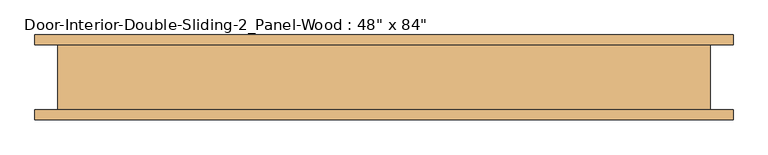
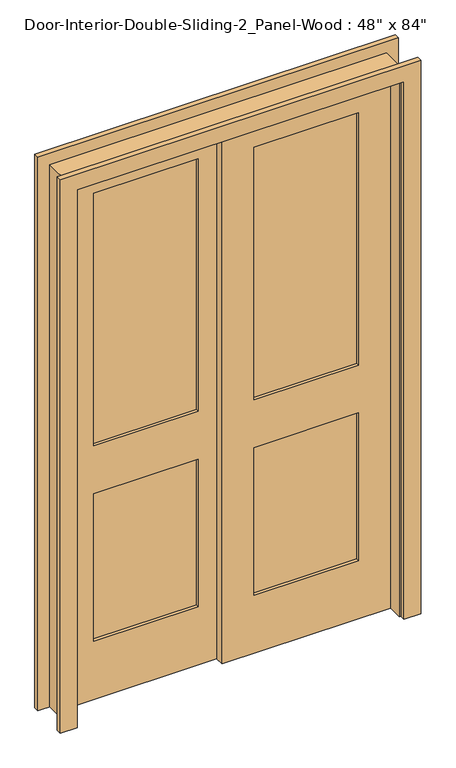
"""IFC4 building model written with IfcOpenShell, lengths in millimetres: door geometry."""

import ifcopenshell
import ifcopenshell.guid

model = None  # the IFC model being written
_history = None  # IfcOwnerHistory: only IFC2X3 demands one
_inside = {}  # id of a spatial element -> (the spatial element, [elements in it])
_under = {}  # id of a project, library or spatial element -> (it, [spatial elements below it])
_declared = {}  # id of a project -> (the project, [libraries it declares])
_typed = {}  # id of a type object -> (the type object, [elements of that type])
_made_of = {}  # id of a material, layer set ... -> (it, [elements and type objects made of it])


def new_model(schema):
    """Start an empty IFC model of exactly this schema.

    Asked for "IFC4X3", IfcOpenShell would pick the latest addendum, in which some entities
    have other attributes; the version numbers below select the first issue.
    IFC2X3 requires an IfcOwnerHistory on every rooted entity: one is made here for all.
    """
    global model, _history
    if schema == "IFC4X3":
        model = ifcopenshell.file(schema_version=(4, 3, 0, 0))
    else:
        model = ifcopenshell.file(schema=schema)
    _inside.clear()
    _under.clear()
    _declared.clear()
    _typed.clear()
    _made_of.clear()
    _history = None
    if model.schema == "IFC2X3":
        org = make("IfcOrganization", Name="unknown")
        user = make(
            "IfcPersonAndOrganization",
            ThePerson=make("IfcPerson", FamilyName="unknown"),
            TheOrganization=org,
        )
        app = make(
            "IfcApplication",
            ApplicationDeveloper=org,
            Version="unknown",
            ApplicationFullName="unknown",
            ApplicationIdentifier="unknown",
        )
        _history = make(
            "IfcOwnerHistory",
            OwningUser=user,
            OwningApplication=app,
            ChangeAction="ADDED",
            CreationDate=0,
        )
    return model


def make(cls, **values):
    """One entity of the class cls with the attributes given. An attribute that is None is left unset."""
    return model.create_entity(
        cls, **{name: value for name, value in values.items() if value is not None}
    )


def rooted(cls, **values):
    """An entity with a GlobalId (a new one), such as an element, a storey or a relation."""
    return make(cls, GlobalId=ifcopenshell.guid.new(), OwnerHistory=_history, **values)


def si_unit(unit_type, name, prefix=None):
    """IfcSIUnit, for example si_unit("LENGTHUNIT", "METRE", prefix="MILLI")."""
    return make("IfcSIUnit", UnitType=unit_type, Prefix=prefix, Name=name)


def assignment(units):
    """IfcUnitAssignment: the units of a project."""
    return None if units is None else make("IfcUnitAssignment", Units=units)


def point(xyz):
    """IfcCartesianPoint."""
    return None if xyz is None else make("IfcCartesianPoint", Coordinates=xyz)


def direction(xyz):
    """IfcDirection."""
    return None if xyz is None else make("IfcDirection", DirectionRatios=xyz)


def frame(location, z_axis=None, x_axis=None):
    """IfcAxis2Placement3D, a coordinate frame: its origin and axes. An axis left out is left unset."""
    return make(
        "IfcAxis2Placement3D",
        Location=point(location),
        Axis=direction(z_axis),
        RefDirection=direction(x_axis),
    )


def origin():
    """The frame at (0, 0, 0) with its axes left unset."""
    return frame((0.0, 0.0, 0.0))


def place(relative_to, where):
    """IfcLocalPlacement: puts the frame where relative to a parent placement (None: the world)."""
    return make(
        "IfcLocalPlacement", PlacementRelTo=relative_to, RelativePlacement=where
    )


def context(
    kind, dimensions, precision=None, world=None, true_north=None, identifier=None
):
    """IfcGeometricRepresentationContext, for example the 3D "Model" context."""
    return make(
        "IfcGeometricRepresentationContext",
        ContextIdentifier=identifier,
        ContextType=kind,
        CoordinateSpaceDimension=dimensions,
        Precision=precision,
        WorldCoordinateSystem=world,
        TrueNorth=true_north,
    )


def project(units=None, contexts=None):
    """IfcProject with its units and contexts."""
    return rooted(
        "IfcProject",
        Name="project",
        RepresentationContexts=contexts,
        UnitsInContext=assignment(units),
    )


def spatial(cls, under=None, at=None, **own):
    """A site, building, storey or space (cls), placed at a placement, below another one or the project."""
    s = rooted(cls, ObjectPlacement=at, **own)
    if under is not None:
        _under.setdefault(under.id(), (under, []))[1].append(s)
    return s


def polyline(points):
    """IfcPolyline through the points."""
    return make("IfcPolyline", Points=[point(p) for p in points])


def outline(outer, holes=None, kind="AREA"):
    """IfcArbitraryClosedProfileDef: a profile drawn as a closed curve; with holes, ...WithVoids."""
    if holes is None:
        return make("IfcArbitraryClosedProfileDef", ProfileType=kind, OuterCurve=outer)
    return make(
        "IfcArbitraryProfileDefWithVoids",
        ProfileType=kind,
        OuterCurve=outer,
        InnerCurves=holes,
    )


def extrude(swept, where, along, depth):
    """IfcExtrudedAreaSolid: the profile swept, set in the frame where, extruded along a direction by depth."""
    return make(
        "IfcExtrudedAreaSolid",
        SweptArea=swept,
        Position=where,
        ExtrudedDirection=direction(along),
        Depth=depth,
    )


def shape(context_of_items, identifier, shape_type, items):
    """IfcShapeRepresentation: the items that make up one representation, for example the "Body"."""
    return make(
        "IfcShapeRepresentation",
        ContextOfItems=context_of_items,
        RepresentationIdentifier=identifier,
        RepresentationType=shape_type,
        Items=items,
    )


def source(mapping_origin, context_of_items, identifier, shape_type, items):
    """IfcRepresentationMap: a shape defined once, which mapped items show again and again."""
    return make(
        "IfcRepresentationMap",
        MappingOrigin=mapping_origin,
        MappedRepresentation=shape(context_of_items, identifier, shape_type, items),
    )


def transform(
    local_origin,
    x_axis=None,
    y_axis=None,
    z_axis=None,
    scale=None,
    scale2=None,
    scale3=None,
    uniform=True,
):
    """IfcCartesianTransformationOperator3D, or its non-uniform kind. x_axis, y_axis, z_axis: its Axis1, 2, 3."""
    if uniform:
        return make(
            "IfcCartesianTransformationOperator3D",
            Axis1=direction(x_axis),
            Axis2=direction(y_axis),
            LocalOrigin=point(local_origin),
            Scale=scale,
            Axis3=direction(z_axis),
        )
    return make(
        "IfcCartesianTransformationOperator3DnonUniform",
        Axis1=direction(x_axis),
        Axis2=direction(y_axis),
        LocalOrigin=point(local_origin),
        Scale=scale,
        Axis3=direction(z_axis),
        Scale2=scale2,
        Scale3=scale3,
    )


def mapped(mapping_source, mapping_target):
    """IfcMappedItem: shows the shape of a source again, moved by a transform."""
    return make(
        "IfcMappedItem", MappingSource=mapping_source, MappingTarget=mapping_target
    )


def made_of(thing, what):
    """Note that an element or type object is made of a material, layer set ...; save() writes the relation."""
    if what is not None:
        _made_of.setdefault(what.id(), (what, []))[1].append(thing)
    return thing


def element(
    cls,
    number,
    at=None,
    inside=None,
    cuts=None,
    type_object=None,
    material=None,
    context=None,
    identifier="Body",
    shape_type=None,
    held_by="IfcProductDefinitionShape",
    body=None,
    shapes=None,
    **own,
):
    """One element of the class cls, such as IfcWall. Its Tag is "e" and its number.

    at: its placement. inside: the storey or other place that contains it. cuts: it is an
    opening in that element (IfcRelVoidsElement). A single representation is given by context,
    identifier, shape_type and body (its items); several are given by shapes. held_by: the class
    of the entity that holds the representations. save() writes the other relations.
    """
    e = rooted(cls, Tag="e%d" % number, ObjectPlacement=at, **own)
    if body is not None:
        shapes = [shape(context, identifier, shape_type, body)]
    if shapes is not None:
        e.Representation = make(held_by, Representations=shapes)
    if inside is not None:
        _inside.setdefault(inside.id(), (inside, []))[1].append(e)
    if cuts is not None:
        rooted(
            "IfcRelVoidsElement", RelatingBuildingElement=cuts, RelatedOpeningElement=e
        )
    if type_object is not None:
        _typed.setdefault(type_object.id(), (type_object, []))[1].append(e)
    return made_of(e, material)


def aggregate(whole, parts):
    """IfcRelAggregates: a whole, such as a stair, and the parts it consists of."""
    return rooted("IfcRelAggregates", RelatingObject=whole, RelatedObjects=parts)


def save(model, path):
    """Write the relations noted so far, then the file.

    IfcRelAggregates (storeys below a building ...), IfcRelContainedInSpatialStructure (elements
    in a storey), IfcRelDefinesByType, IfcRelAssociatesMaterial and IfcRelDeclares: one each for
    every whole, place, type object, material and project.
    """
    for whole, parts in _under.values():
        aggregate(whole, parts)
    for where, things in _inside.values():
        rooted(
            "IfcRelContainedInSpatialStructure",
            RelatedElements=things,
            RelatingStructure=where,
        )
    for kind, things in _typed.values():
        rooted("IfcRelDefinesByType", RelatedObjects=things, RelatingType=kind)
    for what, things in _made_of.values():
        rooted("IfcRelAssociatesMaterial", RelatedObjects=things, RelatingMaterial=what)
    for by, libraries in _declared.values():
        rooted("IfcRelDeclares", RelatingContext=by, RelatedDefinitions=libraries)
    model.write(path)


def door_38ea5fad(model_context):
    return source(origin(), model_context, "Body", "SweptSolid", [
        extrude(outline(polyline([(488.95, 2.1166667), (95.25, 2.1166667), (95.25, 13.7583333), (488.95, 13.7583333), (488.95, 2.1166667)])), frame((0.0, 0.0, 1009.65), z_axis=(0.0, 0.0, 1.0), x_axis=(1.0, 0.0, 0.0)), (0.0, 0.0, 1.0), 1004.8875),
        extrude(outline(polyline([(488.95, 2.1166667), (95.25, 2.1166667), (95.25, 13.7583333), (488.95, 13.7583333), (488.95, 2.1166667)])), frame((0.0, 0.0, 231.775), z_axis=(0.0, 0.0, 1.0), x_axis=(1.0, 0.0, 0.0)), (0.0, 0.0, 1.0), 587.375),
        extrude(outline(polyline([(2133.6, -25.4), (0.0, -25.4), (0.0, 609.6), (2133.6, 609.6), (2133.6, -25.4)]), holes=[polyline([(2014.5375, 95.25), (2014.5375, 488.95), (1009.65, 488.95), (1009.65, 95.25), (2014.5375, 95.25)]), polyline([(819.15, 95.25), (819.15, 488.95), (231.775, 488.95), (231.775, 95.25), (819.15, 95.25)])]), frame((0.0, -9.525, 0.0), z_axis=(0.0, 1.0, 0.0), x_axis=(0.0, 0.0, 1.0)), (0.0, 0.0, 1.0), 34.925),
        extrude(outline(polyline([(-95.25, 37.0416667), (-488.95, 37.0416667), (-488.95, 48.6833333), (-95.25, 48.6833333), (-95.25, 37.0416667)])), frame((0.0, 0.0, 1009.65), z_axis=(0.0, 0.0, 1.0), x_axis=(1.0, 0.0, 0.0)), (0.0, 0.0, 1.0), 1004.8875),
        extrude(outline(polyline([(-95.25, 37.0416667), (-488.95, 37.0416667), (-488.95, 48.6833333), (-95.25, 48.6833333), (-95.25, 37.0416667)])), frame((0.0, 0.0, 231.775), z_axis=(0.0, 0.0, 1.0), x_axis=(1.0, 0.0, 0.0)), (0.0, 0.0, 1.0), 587.375),
        extrude(outline(polyline([(2133.6, -609.6), (0.0, -609.6), (0.0, 25.4), (2133.6, 25.4), (2133.6, -609.6)]), holes=[polyline([(2014.5375, -488.95), (2014.5375, -95.25), (1009.65, -95.25), (1009.65, -488.95), (2014.5375, -488.95)]), polyline([(819.15, -488.95), (819.15, -95.25), (231.775, -95.25), (231.775, -488.95), (819.15, -488.95)])]), frame((0.0, 25.4, 0.0), z_axis=(0.0, 1.0, 0.0), x_axis=(0.0, 0.0, 1.0)), (0.0, 0.0, 1.0), 34.925),
        extrude(outline(polyline([(0.0, 609.6), (0.0, 635.0), (2159.0, 635.0), (2159.0, -635.0), (0.0, -635.0), (0.0, -609.6), (2133.6, -609.6), (2133.6, 609.6), (0.0, 609.6)])), frame((0.0, -66.675, 0.0), z_axis=(0.0, 1.0, 0.0), x_axis=(0.0, 0.0, 1.0)), (0.0, 0.0, 1.0), 127.0),
        extrude(outline(polyline([(0.0, 615.95), (0.0, 679.45), (2203.45, 679.45), (2203.45, -679.45), (0.0, -679.45), (0.0, -615.95), (2139.95, -615.95), (2139.95, 615.95), (0.0, 615.95)])), frame((0.0, -85.725, 0.0), z_axis=(0.0, 1.0, 0.0), x_axis=(0.0, 0.0, 1.0)), (0.0, 0.0, 1.0), 19.05),
        extrude(outline(polyline([(0.0, 615.95), (0.0, 679.45), (2203.45, 679.45), (2203.45, -679.45), (0.0, -679.45), (0.0, -615.95), (2139.95, -615.95), (2139.95, 615.95), (0.0, 615.95)])), frame((0.0, 60.325, 0.0), z_axis=(0.0, 1.0, 0.0), x_axis=(0.0, 0.0, 1.0)), (0.0, 0.0, 1.0), 19.05),
    ])


if __name__ == "__main__":
    model = new_model("IFC4")
    model_context = context("Model", 3, world=origin())
    ifc_project = project(units=[si_unit("LENGTHUNIT", "METRE", prefix="MILLI")], contexts=[model_context])
    site = spatial("IfcSite", under=ifc_project)
    building = spatial("IfcBuilding", under=site)
    placement = place(None, origin())
    door_shape = door_38ea5fad(model_context)
    element("IfcDoor", 1, ObjectType="Door-Interior-Double-Sliding-2_Panel-Wood : 48\" x 84\"", at=placement, inside=building, context=model_context, shape_type="MappedRepresentation", body=[
        mapped(door_shape, transform((0.0, 0.0, 0.0), x_axis=(1.0, 0.0, 0.0), y_axis=(0.0, 1.0, 0.0), z_axis=(0.0, 0.0, 1.0))),
    ])
    save(model, "model.ifc")

# Revit data of these elements
# Type "Door-Interior-Double-Sliding-2_Panel-Wood : 48\" x 84\""
#   Type Mark = "13"
#   Assembly Code = "C1020300"
#   Analytic Construction = "Wooden"
#   Top Rail = 0' - 4 11/16"
#   Thickness = 0' - 1 3/8"
#   Thermal Resistance (R) = 2.5876 (h·ft²·°F)/BTU
#   Stiles = 0' - 4 3/4"
#   Rough Width = 4' - 2"
#   Rough Height = 7' - 1"
#   Lock Rail = 0' - 7 1/2"
#   Height = 7' - 0"
#   Width = 4' - 0"
#   Heat Transfer Coefficient (U) = 0.3865 BTU/(h·ft²·°F)
#   Bottom Rail = 0' - 9 1/8"
#   Function = 0
#   Define Thermal Properties by = 1
#   Trim Material = Cherry
#   Panel Material = Cherry
#   Frame Material = Cherry
#   Visual Light Transmittance = 0
#   Solar Heat Gain Coefficient = 0
#   Wall Closure = (empty or 0)
#   Function = (empty or 0)
# Element 1 (IfcDoor, "Door-Interior-Double-Sliding-2_Panel-Wood : 48\" x 84\"")
#   Materials on its faces: "Cherry"
# Materials
#   "Cherry": class "Wood", colour RGB 157 77 38, transparency 0, Description = "Prunus Serotina", Cost = 0
